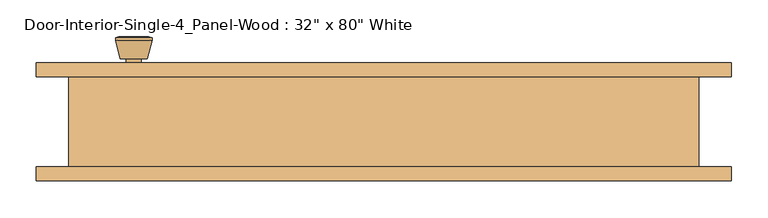
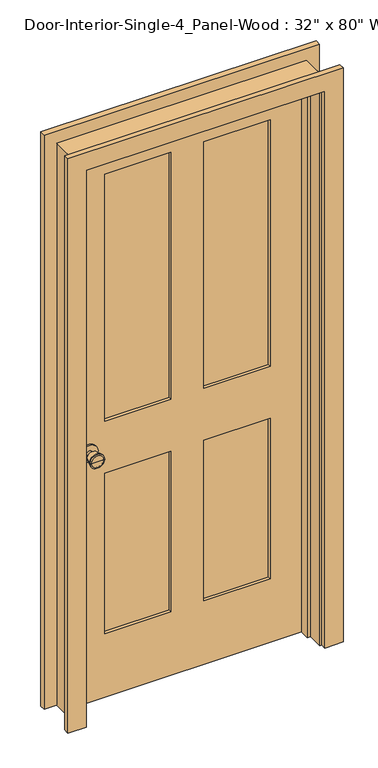
"""IFC4 building model written with IfcOpenShell, lengths in millimetres: door geometry."""

from ifc_helpers import new_model, si_unit, point, frame, frame_2d, origin, place, context, project, spatial, polyline, circle_curve, trimmed, segment, composite_curve, outline, extrude, faceted_brep, source, transform, mapped, element, save
from ifc_brep_helpers import plane_surface, cylinder_surface, revolved_surface, advanced_brep


def door_4f901230(model_context):
    return source(origin(), model_context, "Body", "SolidModel", [
        advanced_brep(
        [(-342.9, 17.8125, 914.4), (-332.9, 17.8125, 914.4), (-352.9, 17.8125, 914.4), (-322.4241324, -31.1875, 914.4), (-342.9, -31.1875, 914.4), (-363.3758676, -31.1875, 914.4), (-317.9, -29.3596319, 914.4), (-367.9, -29.3596319, 914.4), (-317.9, -25.8959537, 914.4), (-367.9, -25.8959537, 914.4), (-324.263764, -1.1875, 914.4), (-361.536236, -1.1875, 914.4), (-332.9, -1.1875, 914.4), (-352.9, -1.1875, 914.4)],
        [
            (0, 1),
            (1, 2, circle_curve(frame((-342.9, 17.8125, 914.4), z_axis=(0.0, 1.0, 0.0), x_axis=(-1.0, 0.0, 0.0)), 10.0)),
            (2, 0),
            (2, 1, circle_curve(frame((-342.9, 17.8125, 914.4), z_axis=(0.0, 1.0, 0.0), x_axis=(-1.0, 0.0, 0.0)), 10.0)),
            (3, 4),
            (4, 5),
            (5, 3, circle_curve(frame((-342.9, -31.1875, 914.4), z_axis=(0.0, -1.0, 0.0), x_axis=(-1.0, 0.0, 0.0)), 20.4758676)),
            (3, 5, circle_curve(frame((-342.9, -31.1875, 914.4), z_axis=(0.0, -1.0, 0.0), x_axis=(-1.0, 0.0, 0.0)), 20.4758676)),
            (6, 3),
            (5, 7),
            (7, 6, circle_curve(frame((-342.9, -29.3596319, 914.4), z_axis=(0.0, -1.0, 0.0), x_axis=(-1.0, 0.0, 0.0)), 25.0)),
            (6, 7, circle_curve(frame((-342.9, -29.3596319, 914.4), z_axis=(0.0, -1.0, 0.0), x_axis=(-1.0, 0.0, 0.0)), 25.0)),
            (8, 6),
            (7, 9),
            (9, 8, circle_curve(frame((-342.9, -25.8959537, 914.4), z_axis=(0.0, -1.0, 0.0), x_axis=(-1.0, 0.0, 0.0)), 25.0)),
            (8, 9, circle_curve(frame((-342.9, -25.8959537, 914.4), z_axis=(0.0, -1.0, 0.0), x_axis=(-1.0, 0.0, 0.0)), 25.0)),
            (10, 8),
            (9, 11),
            (11, 10, circle_curve(frame((-342.9, -1.1875, 914.4), z_axis=(0.0, -1.0, 0.0), x_axis=(-1.0, 0.0, 0.0)), 18.636236)),
            (10, 11, circle_curve(frame((-342.9, -1.1875, 914.4), z_axis=(0.0, -1.0, 0.0), x_axis=(-1.0, 0.0, 0.0)), 18.636236)),
            (12, 10),
            (11, 13),
            (13, 12, circle_curve(frame((-342.9, -1.1875, 914.4), z_axis=(0.0, -1.0, 0.0), x_axis=(-1.0, 0.0, 0.0)), 10.0)),
            (12, 13, circle_curve(frame((-342.9, -1.1875, 914.4), z_axis=(0.0, -1.0, 0.0), x_axis=(-1.0, 0.0, 0.0)), 10.0)),
            (1, 12),
            (13, 2),
        ],
        [
            plane_surface(frame((-342.9, 17.8125, 914.4), z_axis=(0.0, 1.0, 0.0), x_axis=(-1.0, 0.0, 0.0))),
            plane_surface(frame((-342.9, -31.1875, 914.4), z_axis=(0.0, -1.0, 0.0), x_axis=(-1.0, 0.0, 0.0))),
            revolved_surface(polyline([(-363.3758676, -31.1875, 914.4), (-367.9, -29.3596319, 914.4)]), (-342.9, 17.8125, 914.4), (0.0, 1.0, 0.0)),
            cylinder_surface(frame((-342.9, 17.8125, 914.4), z_axis=(0.0, 1.0, 0.0), x_axis=(-1.0, 0.0, 0.0)), 25.0),
            revolved_surface(polyline([(-367.9, -25.8959537, 914.4), (-361.536236, -1.1875, 914.4)]), (-342.9, 17.8125, 914.4), (0.0, 1.0, 0.0)),
            plane_surface(frame((-342.9, -1.1875, 914.4), z_axis=(0.0, 1.0, 0.0), x_axis=(-1.0, 0.0, 0.0))),
            cylinder_surface(frame((-342.9, 17.8125, 914.4), z_axis=(0.0, 1.0, 0.0), x_axis=(-1.0, 0.0, 0.0)), 10.0),
        ],
        [
            (0, [[1, 2, 3]]),
            (0, [[-3, 4, -1]]),
            (1, [[5, 6, 7]]),
            (1, [[-6, -5, 8]]),
            (2, [[9, -7, 10, 11]]),
            (2, [[-10, -8, -9, 12]]),
            (3, [[13, -11, 14, 15]]),
            (3, [[-14, -12, -13, 16]]),
            (4, [[17, -15, 18, 19]]),
            (4, [[-18, -16, -17, 20]]),
            (5, [[21, -19, 22, 23]]),
            (5, [[-22, -20, -21, 24]]),
            (6, [[25, -23, 26, -2]]),
            (6, [[-26, -24, -25, -4]]),
        ],
    ),
        extrude(outline(composite_curve([segment(trimmed(circle_curve(frame_2d((914.4, -342.9)), 30.0), [point((914.4, -372.9))], [point((914.4, -312.9))], False, "CARTESIAN"), True, "CONTINUOUS"), segment(trimmed(circle_curve(frame_2d((914.4, -342.9)), 30.0), [point((914.4, -312.9))], [point((914.4, -372.9))], False, "CARTESIAN"), True, "CONTINUOUS")], self_intersect=False)), frame((0.0, 17.8125, 0.0), z_axis=(0.0, 1.0, 0.0), x_axis=(0.0, 0.0, 1.0)), (0.0, 0.0, 1.0), 6.0),
        advanced_brep(
        [(-342.9, 64.7375, 914.4), (-352.9, 64.7375, 914.4), (-332.9, 64.7375, 914.4), (-322.4241324, 113.7375, 914.4), (-363.3758676, 113.7375, 914.4), (-342.9, 113.7375, 914.4), (-317.9, 111.9096319, 914.4), (-367.9, 111.9096319, 914.4), (-317.9, 108.4459537, 914.4), (-367.9, 108.4459537, 914.4), (-324.263764, 83.7375, 914.4), (-361.536236, 83.7375, 914.4), (-332.9, 83.7375, 914.4), (-352.9, 83.7375, 914.4)],
        [
            (0, 1),
            (1, 2, circle_curve(frame((-342.9, 64.7375, 914.4), z_axis=(0.0, -1.0, 0.0), x_axis=(-1.0, 0.0, 0.0)), 10.0)),
            (2, 0),
            (2, 1, circle_curve(frame((-342.9, 64.7375, 914.4), z_axis=(0.0, -1.0, 0.0), x_axis=(-1.0, 0.0, 0.0)), 10.0)),
            (3, 4, circle_curve(frame((-342.9, 113.7375, 914.4), z_axis=(0.0, 1.0, 0.0), x_axis=(-1.0, 0.0, 0.0)), 20.4758676)),
            (4, 5),
            (5, 3),
            (4, 3, circle_curve(frame((-342.9, 113.7375, 914.4), z_axis=(0.0, 1.0, 0.0), x_axis=(-1.0, 0.0, 0.0)), 20.4758676)),
            (6, 7, circle_curve(frame((-342.9, 111.9096319, 914.4), z_axis=(0.0, 1.0, 0.0), x_axis=(-1.0, 0.0, 0.0)), 25.0)),
            (7, 4),
            (3, 6),
            (7, 6, circle_curve(frame((-342.9, 111.9096319, 914.4), z_axis=(0.0, 1.0, 0.0), x_axis=(-1.0, 0.0, 0.0)), 25.0)),
            (8, 9, circle_curve(frame((-342.9, 108.4459537, 914.4), z_axis=(0.0, 1.0, 0.0), x_axis=(-1.0, 0.0, 0.0)), 25.0)),
            (9, 7),
            (6, 8),
            (9, 8, circle_curve(frame((-342.9, 108.4459537, 914.4), z_axis=(0.0, 1.0, 0.0), x_axis=(-1.0, 0.0, 0.0)), 25.0)),
            (10, 11, circle_curve(frame((-342.9, 83.7375, 914.4), z_axis=(0.0, 1.0, 0.0), x_axis=(-1.0, 0.0, 0.0)), 18.636236)),
            (11, 9),
            (8, 10),
            (11, 10, circle_curve(frame((-342.9, 83.7375, 914.4), z_axis=(0.0, 1.0, 0.0), x_axis=(-1.0, 0.0, 0.0)), 18.636236)),
            (12, 13, circle_curve(frame((-342.9, 83.7375, 914.4), z_axis=(0.0, 1.0, 0.0), x_axis=(-1.0, 0.0, 0.0)), 10.0)),
            (13, 11),
            (10, 12),
            (13, 12, circle_curve(frame((-342.9, 83.7375, 914.4), z_axis=(0.0, 1.0, 0.0), x_axis=(-1.0, 0.0, 0.0)), 10.0)),
            (1, 13),
            (12, 2),
        ],
        [
            plane_surface(frame((-342.9, 64.7375, 914.4), z_axis=(0.0, -1.0, 0.0), x_axis=(-1.0, 0.0, 0.0))),
            plane_surface(frame((-342.9, 113.7375, 914.4), z_axis=(0.0, 1.0, 0.0), x_axis=(-1.0, 0.0, 0.0))),
            revolved_surface(polyline([(-363.3758676, 113.7375, 914.4), (-367.9, 111.9096319, 914.4)]), (-342.9, 64.7375, 914.4), (0.0, -1.0, 0.0)),
            cylinder_surface(frame((-342.9, 64.7375, 914.4), z_axis=(0.0, -1.0, 0.0), x_axis=(-1.0, 0.0, 0.0)), 25.0),
            revolved_surface(polyline([(-367.9, 108.4459537, 914.4), (-361.536236, 83.7375, 914.4)]), (-342.9, 64.7375, 914.4), (0.0, -1.0, 0.0)),
            plane_surface(frame((-342.9, 83.7375, 914.4), z_axis=(0.0, -1.0, 0.0), x_axis=(-1.0, 0.0, 0.0))),
            cylinder_surface(frame((-342.9, 64.7375, 914.4), z_axis=(0.0, -1.0, 0.0), x_axis=(-1.0, 0.0, 0.0)), 10.0),
        ],
        [
            (0, [[1, 2, 3]]),
            (0, [[-3, 4, -1]]),
            (1, [[5, 6, 7]]),
            (1, [[8, -7, -6]]),
            (2, [[9, 10, -5, 11]]),
            (2, [[12, -11, -8, -10]]),
            (3, [[13, 14, -9, 15]]),
            (3, [[16, -15, -12, -14]]),
            (4, [[17, 18, -13, 19]]),
            (4, [[20, -19, -16, -18]]),
            (5, [[21, 22, -17, 23]]),
            (5, [[24, -23, -20, -22]]),
            (6, [[-2, 25, -21, 26]]),
            (6, [[-4, -26, -24, -25]]),
        ],
    ),
        extrude(outline(composite_curve([segment(trimmed(circle_curve(frame_2d((914.4, -342.9)), 30.0), [point((914.4, -372.9))], [point((914.4, -312.9))], False, "CARTESIAN"), True, "CONTINUOUS"), segment(trimmed(circle_curve(frame_2d((914.4, -342.9)), 30.0), [point((914.4, -312.9))], [point((914.4, -372.9))], False, "CARTESIAN"), True, "CONTINUOUS")], self_intersect=False)), frame((0.0, 58.7375, 0.0), z_axis=(0.0, 1.0, 0.0), x_axis=(0.0, 0.0, 1.0)), (0.0, 0.0, 1.0), 6.0),
        extrude(outline(polyline([(285.75, 35.4541667), (57.15, 35.4541667), (57.15, 47.0958333), (285.75, 47.0958333), (285.75, 35.4541667)])), frame((0.0, 0.0, 1009.65), z_axis=(0.0, 0.0, 1.0), x_axis=(1.0, 0.0, 0.0)), (0.0, 0.0, 1.0), 903.2875),
        extrude(outline(polyline([(-57.15, 35.4541667), (-285.75, 35.4541667), (-285.75, 47.0958333), (-57.15, 47.0958333), (-57.15, 35.4541667)])), frame((0.0, 0.0, 1009.65), z_axis=(0.0, 0.0, 1.0), x_axis=(1.0, 0.0, 0.0)), (0.0, 0.0, 1.0), 903.2875),
        extrude(outline(polyline([(285.75, 35.4541667), (57.15, 35.4541667), (57.15, 47.0958333), (285.75, 47.0958333), (285.75, 35.4541667)])), frame((0.0, 0.0, 231.775), z_axis=(0.0, 0.0, 1.0), x_axis=(1.0, 0.0, 0.0)), (0.0, 0.0, 1.0), 587.375),
        extrude(outline(polyline([(-57.15, 35.4541667), (-285.75, 35.4541667), (-285.75, 47.0958333), (-57.15, 47.0958333), (-57.15, 35.4541667)])), frame((0.0, 0.0, 231.775), z_axis=(0.0, 0.0, 1.0), x_axis=(1.0, 0.0, 0.0)), (0.0, 0.0, 1.0), 587.375),
        extrude(outline(polyline([(2032.0, -406.4), (0.0, -406.4), (0.0, 406.4), (2032.0, 406.4), (2032.0, -406.4)]), holes=[polyline([(1912.9375, 57.15), (1912.9375, 285.75), (1009.65, 285.75), (1009.65, 57.15), (1912.9375, 57.15)]), polyline([(1009.65, -57.15), (1009.65, -285.75), (1912.9375, -285.75), (1912.9375, -57.15), (1009.65, -57.15)]), polyline([(819.15, 57.15), (819.15, 285.75), (231.775, 285.75), (231.775, 57.15), (819.15, 57.15)]), polyline([(231.775, -57.15), (231.775, -285.75), (819.15, -285.75), (819.15, -57.15), (231.775, -57.15)])]), frame((0.0, 23.8125, 0.0), z_axis=(0.0, 1.0, 0.0), x_axis=(0.0, 0.0, 1.0)), (0.0, 0.0, 1.0), 34.925),
        faceted_brep([(431.8, 58.7375, 0.0), (431.8, -65.0875, 0.0), (406.4, -65.0875, 0.0), (406.4, -11.1125, 0.0), (393.7, -11.1125, 0.0), (393.7, 23.8125, 0.0), (406.4, 23.8125, 0.0), (406.4, 58.7375, 0.0), (431.8, 58.7375, 2057.4), (431.8, -65.0875, 2057.4), (-431.8, -65.0875, 2057.4), (-431.8, -65.0875, 0.0), (-406.4, -65.0875, 0.0), (-406.4, -65.0875, 2032.0), (406.4, -65.0875, 2032.0), (406.4, -11.1125, 2032.0), (-406.4, -11.1125, 2032.0), (-406.4, -11.1125, 0.0), (-393.7, -11.1125, 0.0), (-393.7, -11.1125, 2019.3), (393.7, -11.1125, 2019.3), (393.7, 23.8125, 2019.3), (-393.7, 23.8125, 2019.3), (-393.7, 23.8125, 0.0), (-406.4, 23.8125, 0.0), (-406.4, 23.8125, 2032.0), (406.4, 23.8125, 2032.0), (406.4, 58.7375, 2032.0), (-406.4, 58.7375, 2032.0), (-406.4, 58.7375, 0.0), (-431.8, 58.7375, 0.0), (-431.8, 58.7375, 2057.4)], [[[0, 1, 2, 3, 4, 5, 6, 7]], [[1, 0, 8, 9]], [[2, 1, 9, 10, 11, 12, 13, 14]], [[3, 2, 14, 15]], [[4, 3, 15, 16, 17, 18, 19, 20]], [[5, 4, 20, 21]], [[6, 5, 21, 22, 23, 24, 25, 26]], [[7, 6, 26, 27]], [[0, 7, 27, 28, 29, 30, 31, 8]], [[9, 8, 31, 10]], [[15, 14, 13, 16]], [[21, 20, 19, 22]], [[27, 26, 25, 28]], [[30, 29, 24, 23, 18, 17, 12, 11]], [[10, 31, 30, 11]], [[16, 13, 12, 17]], [[22, 19, 18, 23]], [[28, 25, 24, 29]]]),
        extrude(outline(polyline([(0.0, 412.75), (0.0, 476.25), (2101.85, 476.25), (2101.85, -476.25), (0.0, -476.25), (0.0, -412.75), (2038.35, -412.75), (2038.35, 412.75), (0.0, 412.75)])), frame((0.0, -84.1375, 0.0), z_axis=(0.0, 1.0, 0.0), x_axis=(0.0, 0.0, 1.0)), (0.0, 0.0, 1.0), 19.05),
        extrude(outline(polyline([(0.0, 412.75), (0.0, 476.25), (2101.85, 476.25), (2101.85, -476.25), (0.0, -476.25), (0.0, -412.75), (2038.35, -412.75), (2038.35, 412.75), (0.0, 412.75)])), frame((0.0, 58.7375, 0.0), z_axis=(0.0, 1.0, 0.0), x_axis=(0.0, 0.0, 1.0)), (0.0, 0.0, 1.0), 19.05),
    ])


if __name__ == "__main__":
    model = new_model("IFC4")
    model_context = context("Model", 3, world=origin())
    ifc_project = project(units=[si_unit("LENGTHUNIT", "METRE", prefix="MILLI")], contexts=[model_context])
    site = spatial("IfcSite", under=ifc_project)
    building = spatial("IfcBuilding", under=site)
    placement = place(None, origin())
    door_shape = door_4f901230(model_context)
    element("IfcDoor", 1, ObjectType="Door-Interior-Single-4_Panel-Wood : 32\" x 80\" White", at=placement, inside=building, context=model_context, shape_type="MappedRepresentation", body=[
        mapped(door_shape, transform((0.0, 0.0, 0.0), x_axis=(1.0, 0.0, 0.0), y_axis=(0.0, 1.0, 0.0), z_axis=(0.0, 0.0, 1.0))),
    ])
    save(model, "model.ifc")

# Revit data of these elements
# Type "Door-Interior-Single-4_Panel-Wood : 32\" x 80\" White"
#   Type Mark = "48"
#   COBie.Type.CreatedBy = "doug.wood@us.ibm.com"
#   COBie.Type.CreatedOn = "2016-04-14T02:07:24"
#   COBie.Type.Name = "Doors_Door-Interior-Single-4_Panel-Wood_32\" x 80\" White_48"
#   COBie.Type.Category = "23-30 10 00 : Doors"
#   COBie.Type.Description = "Door-Interior-Single-4_Panel-Wood_32\" x 80\" White"
#   COBie.Type.Manufacturer = ""
#   COBie.Type.ModelNumber = ""
#   Assembly Code = "C1020300"
#   Analytic Construction = "Wooden"
#   COBie.Type.ReplacementCost = 0
#   Top Rail = 0' - 4 11/16"
#   Thickness = 0' - 1 3/8"
#   Thermal Resistance (R) = 0.455703 (m²·K)/W
#   Swing Angle [instance default] = 90.00°
#   Stiles = 0' - 4 3/4"
#   Rough Width = 2' - 10"
#   Rough Height = 6' - 9"
#   Mullion = 0' - 4 1/2"
#   Lock Rail = 0' - 7 1/2"
#   Height = 6' - 8"
#   Width = 2' - 8"
#   Heat Transfer Coefficient (U) = 2.19465 W/(m²·K)
#   Bottom Rail = 0' - 9 1/8"
#   COBie.Type = no
#   Trim Material = Trim - White
#   Panel Material = Door - Panel - White
#   Frame Material = Door - Panel - White
#   Door Handle Material = ARCAT - Metal - Brass, Polished
#   Visual Light Transmittance = 0
#   Solar Heat Gain Coefficient = 0
#   Wall Closure = (empty or 0)
#   Function = (empty or 0)
# Element 1 (IfcDoor, "Door-Interior-Single-4_Panel-Wood : 32\" x 80\" White")
#   Materials on its faces: "Door - Panel - White", "ARCAT - Metal - Brass, Polished", "Trim - White"
# Materials
#   "Trim - White": class "Wood", colour RGB 255 255 255, transparency 0, Cost = 0
#   "Door - Panel - White": class "Wood", colour RGB 255 255 255, transparency 0, Cost = 0
#   "ARCAT - Metal - Brass, Polished": class "Unassigned", colour RGB 246 240 166, transparency 0, Keynote = "05050", Model = "Generic", Manufacturer = "Generic", Description = "Steel, Chrome Plated"
